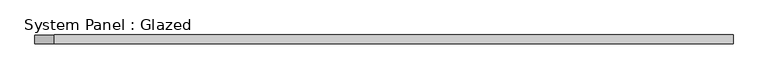
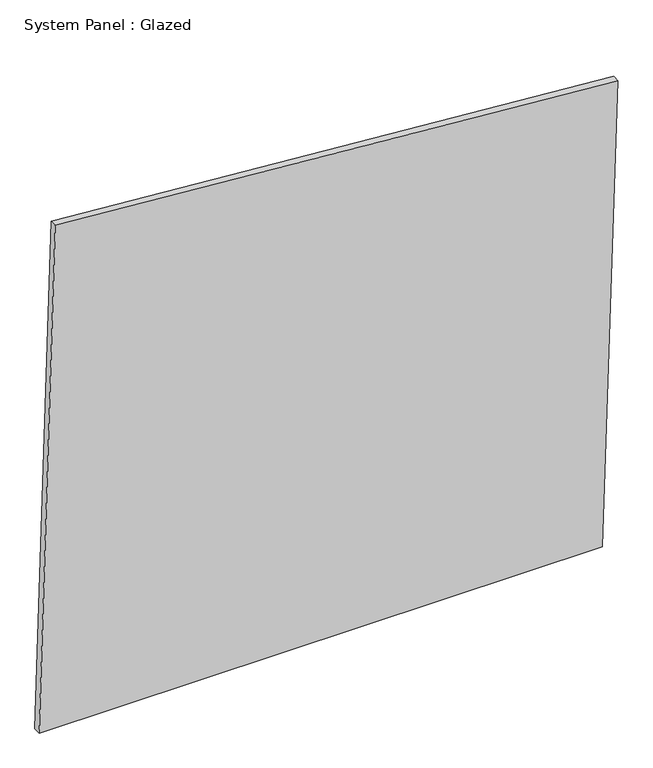
"""IFC4 building model written with IfcOpenShell, lengths in millimetres: plate geometry, System Panel : Glazed."""

from ifc_helpers import new_model, si_unit, frame, origin, place, context, project, spatial, polyline, outline, extrude, source, transform, mapped, element, save


def system_panel_glazed_53210cc6(model_context):
    return source(origin(), model_context, "Body", "SweptSolid", [
        extrude(outline(polyline([(0.0, -1001.8989904), (0.0, 947.931492), (1687.1996383, 1001.8989904), (1838.9666874, -946.0465604), (0.0, -1001.8989904)])), frame((0.0, -49.5, 0.0), z_axis=(0.0, 1.0, 0.0), x_axis=(0.0, 0.0, 1.0)), (0.0, 0.0, 1.0), 25.0),
    ])


if __name__ == "__main__":
    model = new_model("IFC4")
    model_context = context("Model", 3, world=origin())
    ifc_project = project(units=[si_unit("LENGTHUNIT", "METRE", prefix="MILLI")], contexts=[model_context])
    site = spatial("IfcSite", under=ifc_project)
    building = spatial("IfcBuilding", under=site)
    placement = place(None, origin())
    system_panel_glazed_shape = system_panel_glazed_53210cc6(model_context)
    element("IfcPlate", 1, ObjectType="System Panel : Glazed", at=placement, inside=building, context=model_context, shape_type="MappedRepresentation", body=[
        mapped(system_panel_glazed_shape, transform((0.0, 0.0, 0.0), x_axis=(1.0, 0.0, 0.0), y_axis=(0.0, 1.0, 0.0), z_axis=(0.0, 0.0, 1.0))),
    ])
    save(model, "model.ifc")

# Revit data of these elements
# Element 1 (IfcPlate, "System Panel : Glazed")
#   Materials on its faces: "Glass, Clear Glazing"
# Materials
#   "Glass, Clear Glazing": class "Glass", colour RGB 247 249 248, transparency 0.85, Description = "Clear glazing", Cost = 0
